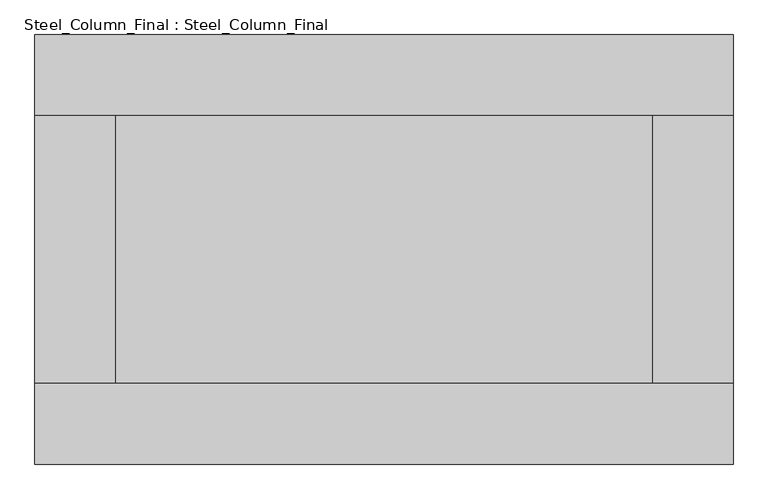
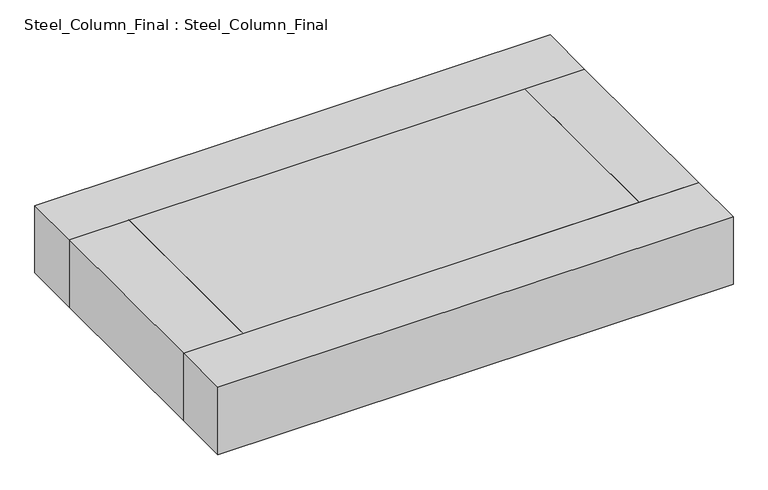
"""IFC4 building model written with IfcOpenShell, lengths in millimetres: proxy geometry, Steel_Column_Final : Steel_Column_Final."""

import ifcopenshell
import ifcopenshell.guid

model = None  # the IFC model being written
_history = None  # IfcOwnerHistory: only IFC2X3 demands one
_inside = {}  # id of a spatial element -> (the spatial element, [elements in it])
_under = {}  # id of a project, library or spatial element -> (it, [spatial elements below it])
_declared = {}  # id of a project -> (the project, [libraries it declares])
_typed = {}  # id of a type object -> (the type object, [elements of that type])
_made_of = {}  # id of a material, layer set ... -> (it, [elements and type objects made of it])


def new_model(schema):
    """Start an empty IFC model of exactly this schema.

    Asked for "IFC4X3", IfcOpenShell would pick the latest addendum, in which some entities
    have other attributes; the version numbers below select the first issue.
    IFC2X3 requires an IfcOwnerHistory on every rooted entity: one is made here for all.
    """
    global model, _history
    if schema == "IFC4X3":
        model = ifcopenshell.file(schema_version=(4, 3, 0, 0))
    else:
        model = ifcopenshell.file(schema=schema)
    _inside.clear()
    _under.clear()
    _declared.clear()
    _typed.clear()
    _made_of.clear()
    _history = None
    if model.schema == "IFC2X3":
        org = make("IfcOrganization", Name="unknown")
        user = make(
            "IfcPersonAndOrganization",
            ThePerson=make("IfcPerson", FamilyName="unknown"),
            TheOrganization=org,
        )
        app = make(
            "IfcApplication",
            ApplicationDeveloper=org,
            Version="unknown",
            ApplicationFullName="unknown",
            ApplicationIdentifier="unknown",
        )
        _history = make(
            "IfcOwnerHistory",
            OwningUser=user,
            OwningApplication=app,
            ChangeAction="ADDED",
            CreationDate=0,
        )
    return model


def make(cls, **values):
    """One entity of the class cls with the attributes given. An attribute that is None is left unset."""
    return model.create_entity(
        cls, **{name: value for name, value in values.items() if value is not None}
    )


def rooted(cls, **values):
    """An entity with a GlobalId (a new one), such as an element, a storey or a relation."""
    return make(cls, GlobalId=ifcopenshell.guid.new(), OwnerHistory=_history, **values)


def si_unit(unit_type, name, prefix=None):
    """IfcSIUnit, for example si_unit("LENGTHUNIT", "METRE", prefix="MILLI")."""
    return make("IfcSIUnit", UnitType=unit_type, Prefix=prefix, Name=name)


def assignment(units):
    """IfcUnitAssignment: the units of a project."""
    return None if units is None else make("IfcUnitAssignment", Units=units)


def point(xyz):
    """IfcCartesianPoint."""
    return None if xyz is None else make("IfcCartesianPoint", Coordinates=xyz)


def direction(xyz):
    """IfcDirection."""
    return None if xyz is None else make("IfcDirection", DirectionRatios=xyz)


def frame(location, z_axis=None, x_axis=None):
    """IfcAxis2Placement3D, a coordinate frame: its origin and axes. An axis left out is left unset."""
    return make(
        "IfcAxis2Placement3D",
        Location=point(location),
        Axis=direction(z_axis),
        RefDirection=direction(x_axis),
    )


def origin():
    """The frame at (0, 0, 0) with its axes left unset."""
    return frame((0.0, 0.0, 0.0))


def place(relative_to, where):
    """IfcLocalPlacement: puts the frame where relative to a parent placement (None: the world)."""
    return make(
        "IfcLocalPlacement", PlacementRelTo=relative_to, RelativePlacement=where
    )


def context(
    kind, dimensions, precision=None, world=None, true_north=None, identifier=None
):
    """IfcGeometricRepresentationContext, for example the 3D "Model" context."""
    return make(
        "IfcGeometricRepresentationContext",
        ContextIdentifier=identifier,
        ContextType=kind,
        CoordinateSpaceDimension=dimensions,
        Precision=precision,
        WorldCoordinateSystem=world,
        TrueNorth=true_north,
    )


def project(units=None, contexts=None):
    """IfcProject with its units and contexts."""
    return rooted(
        "IfcProject",
        Name="project",
        RepresentationContexts=contexts,
        UnitsInContext=assignment(units),
    )


def spatial(cls, under=None, at=None, **own):
    """A site, building, storey or space (cls), placed at a placement, below another one or the project."""
    s = rooted(cls, ObjectPlacement=at, **own)
    if under is not None:
        _under.setdefault(under.id(), (under, []))[1].append(s)
    return s


def polyline(points):
    """IfcPolyline through the points."""
    return make("IfcPolyline", Points=[point(p) for p in points])


def outline(outer, holes=None, kind="AREA"):
    """IfcArbitraryClosedProfileDef: a profile drawn as a closed curve; with holes, ...WithVoids."""
    if holes is None:
        return make("IfcArbitraryClosedProfileDef", ProfileType=kind, OuterCurve=outer)
    return make(
        "IfcArbitraryProfileDefWithVoids",
        ProfileType=kind,
        OuterCurve=outer,
        InnerCurves=holes,
    )


def extrude(swept, where, along, depth):
    """IfcExtrudedAreaSolid: the profile swept, set in the frame where, extruded along a direction by depth."""
    return make(
        "IfcExtrudedAreaSolid",
        SweptArea=swept,
        Position=where,
        ExtrudedDirection=direction(along),
        Depth=depth,
    )


def shape(context_of_items, identifier, shape_type, items):
    """IfcShapeRepresentation: the items that make up one representation, for example the "Body"."""
    return make(
        "IfcShapeRepresentation",
        ContextOfItems=context_of_items,
        RepresentationIdentifier=identifier,
        RepresentationType=shape_type,
        Items=items,
    )


def source(mapping_origin, context_of_items, identifier, shape_type, items):
    """IfcRepresentationMap: a shape defined once, which mapped items show again and again."""
    return make(
        "IfcRepresentationMap",
        MappingOrigin=mapping_origin,
        MappedRepresentation=shape(context_of_items, identifier, shape_type, items),
    )


def transform(
    local_origin,
    x_axis=None,
    y_axis=None,
    z_axis=None,
    scale=None,
    scale2=None,
    scale3=None,
    uniform=True,
):
    """IfcCartesianTransformationOperator3D, or its non-uniform kind. x_axis, y_axis, z_axis: its Axis1, 2, 3."""
    if uniform:
        return make(
            "IfcCartesianTransformationOperator3D",
            Axis1=direction(x_axis),
            Axis2=direction(y_axis),
            LocalOrigin=point(local_origin),
            Scale=scale,
            Axis3=direction(z_axis),
        )
    return make(
        "IfcCartesianTransformationOperator3DnonUniform",
        Axis1=direction(x_axis),
        Axis2=direction(y_axis),
        LocalOrigin=point(local_origin),
        Scale=scale,
        Axis3=direction(z_axis),
        Scale2=scale2,
        Scale3=scale3,
    )


def mapped(mapping_source, mapping_target):
    """IfcMappedItem: shows the shape of a source again, moved by a transform."""
    return make(
        "IfcMappedItem", MappingSource=mapping_source, MappingTarget=mapping_target
    )


def made_of(thing, what):
    """Note that an element or type object is made of a material, layer set ...; save() writes the relation."""
    if what is not None:
        _made_of.setdefault(what.id(), (what, []))[1].append(thing)
    return thing


def element(
    cls,
    number,
    at=None,
    inside=None,
    cuts=None,
    type_object=None,
    material=None,
    context=None,
    identifier="Body",
    shape_type=None,
    held_by="IfcProductDefinitionShape",
    body=None,
    shapes=None,
    **own,
):
    """One element of the class cls, such as IfcWall. Its Tag is "e" and its number.

    at: its placement. inside: the storey or other place that contains it. cuts: it is an
    opening in that element (IfcRelVoidsElement). A single representation is given by context,
    identifier, shape_type and body (its items); several are given by shapes. held_by: the class
    of the entity that holds the representations. save() writes the other relations.
    """
    e = rooted(cls, Tag="e%d" % number, ObjectPlacement=at, **own)
    if body is not None:
        shapes = [shape(context, identifier, shape_type, body)]
    if shapes is not None:
        e.Representation = make(held_by, Representations=shapes)
    if inside is not None:
        _inside.setdefault(inside.id(), (inside, []))[1].append(e)
    if cuts is not None:
        rooted(
            "IfcRelVoidsElement", RelatingBuildingElement=cuts, RelatedOpeningElement=e
        )
    if type_object is not None:
        _typed.setdefault(type_object.id(), (type_object, []))[1].append(e)
    return made_of(e, material)


def aggregate(whole, parts):
    """IfcRelAggregates: a whole, such as a stair, and the parts it consists of."""
    return rooted("IfcRelAggregates", RelatingObject=whole, RelatedObjects=parts)


def save(model, path):
    """Write the relations noted so far, then the file.

    IfcRelAggregates (storeys below a building ...), IfcRelContainedInSpatialStructure (elements
    in a storey), IfcRelDefinesByType, IfcRelAssociatesMaterial and IfcRelDeclares: one each for
    every whole, place, type object, material and project.
    """
    for whole, parts in _under.values():
        aggregate(whole, parts)
    for where, things in _inside.values():
        rooted(
            "IfcRelContainedInSpatialStructure",
            RelatedElements=things,
            RelatingStructure=where,
        )
    for kind, things in _typed.values():
        rooted("IfcRelDefinesByType", RelatedObjects=things, RelatingType=kind)
    for what, things in _made_of.values():
        rooted("IfcRelAssociatesMaterial", RelatedObjects=things, RelatingMaterial=what)
    for by, libraries in _declared.values():
        rooted("IfcRelDeclares", RelatingContext=by, RelatedDefinitions=libraries)
    model.write(path)


def steel_column_final_steel_column_final_07a735ce(model_context):
    return source(origin(), model_context, "Body", "SweptSolid", [
        extrude(outline(polyline([(6500.0, 2500.0), (-6500.0, 2500.0), (-6500.0, 4000.0), (6500.0, 4000.0), (6500.0, 2500.0)])), frame((0.0, 0.0, 22790.0), z_axis=(0.0, 0.0, 1.0), x_axis=(1.0, 0.0, 0.0)), (0.0, 0.0, 1.0), 1800.0),
        extrude(outline(polyline([(-6500.0, -2500.0), (6500.0, -2500.0), (6500.0, -4000.0), (-6500.0, -4000.0), (-6500.0, -2500.0)])), frame((0.0, 0.0, 22790.0), z_axis=(0.0, 0.0, 1.0), x_axis=(1.0, 0.0, 0.0)), (0.0, 0.0, 1.0), 1800.0),
        extrude(outline(polyline([(5000.0, -2500.0), (5000.0, 2500.0), (6500.0, 2500.0), (6500.0, -2500.0), (5000.0, -2500.0)])), frame((0.0, 0.0, 22790.0), z_axis=(0.0, 0.0, 1.0), x_axis=(1.0, 0.0, 0.0)), (0.0, 0.0, 1.0), 1800.0),
        extrude(outline(polyline([(-5000.0, 2500.0), (-5000.0, -2500.0), (-6500.0, -2500.0), (-6500.0, 2500.0), (-5000.0, 2500.0)])), frame((0.0, 0.0, 22790.0), z_axis=(0.0, 0.0, 1.0), x_axis=(1.0, 0.0, 0.0)), (0.0, 0.0, 1.0), 1800.0),
        extrude(outline(polyline([(-5000.0, -2500.0), (-5000.0, 2500.0), (5000.0, 2500.0), (5000.0, -2500.0), (-5000.0, -2500.0)])), frame((0.0, 0.0, 22790.0), z_axis=(0.0, 0.0, 1.0), x_axis=(1.0, 0.0, 0.0)), (0.0, 0.0, 1.0), 1800.0),
    ])


if __name__ == "__main__":
    model = new_model("IFC4")
    model_context = context("Model", 3, world=origin())
    ifc_project = project(units=[si_unit("LENGTHUNIT", "METRE", prefix="MILLI")], contexts=[model_context])
    site = spatial("IfcSite", under=ifc_project)
    building = spatial("IfcBuilding", under=site)
    placement = place(None, origin())
    steel_column_final_steel_column_final_shape = steel_column_final_steel_column_final_07a735ce(model_context)
    element("IfcBuildingElementProxy", 1, Name="Steel_Column_Final : Steel_Column_Final", ObjectType="Steel_Column_Final : Steel_Column_Final", at=placement, inside=building, context=model_context, shape_type="MappedRepresentation", body=[
        mapped(steel_column_final_steel_column_final_shape, transform((0.0, 0.0, 0.0), x_axis=(1.0, 0.0, 0.0), y_axis=(0.0, 1.0, 0.0), z_axis=(0.0, 0.0, 1.0))),
    ])
    save(model, "model.ifc")

# Revit data of these elements
# Type "Steel_Column_Final : Steel_Column_Final"
#   Top Width [instance default] = 5000 mm
#   Top Length = 10000 mm
#   Length = 21000 mm
#   Height [instance default] = 50000 mm
#   Bottom Width [instance default] = 5000 mm
#   Default Elevation = 0
# Element 1 (IfcBuildingElementProxy, "Steel_Column_Final : Steel_Column_Final")
#   Height = 22790 mm
